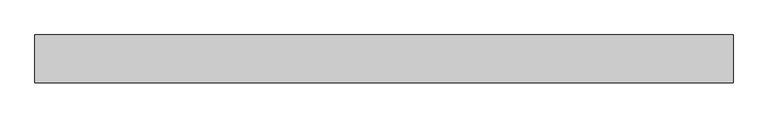
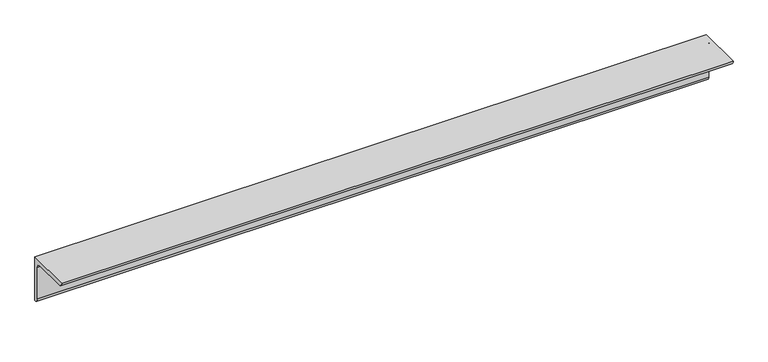
"""IFC4 building model written with IfcOpenShell, lengths in millimetres: member geometry, 0912_Steel Framing_L-KSD3502 : H_SB_AR_S03_L-130x130x12_HBR3."""

import ifcopenshell
import ifcopenshell.guid

model = None  # the IFC model being written
_history = None  # IfcOwnerHistory: only IFC2X3 demands one
_inside = {}  # id of a spatial element -> (the spatial element, [elements in it])
_under = {}  # id of a project, library or spatial element -> (it, [spatial elements below it])
_declared = {}  # id of a project -> (the project, [libraries it declares])
_typed = {}  # id of a type object -> (the type object, [elements of that type])
_made_of = {}  # id of a material, layer set ... -> (it, [elements and type objects made of it])


def new_model(schema):
    """Start an empty IFC model of exactly this schema.

    Asked for "IFC4X3", IfcOpenShell would pick the latest addendum, in which some entities
    have other attributes; the version numbers below select the first issue.
    IFC2X3 requires an IfcOwnerHistory on every rooted entity: one is made here for all.
    """
    global model, _history
    if schema == "IFC4X3":
        model = ifcopenshell.file(schema_version=(4, 3, 0, 0))
    else:
        model = ifcopenshell.file(schema=schema)
    _inside.clear()
    _under.clear()
    _declared.clear()
    _typed.clear()
    _made_of.clear()
    _history = None
    if model.schema == "IFC2X3":
        org = make("IfcOrganization", Name="unknown")
        user = make(
            "IfcPersonAndOrganization",
            ThePerson=make("IfcPerson", FamilyName="unknown"),
            TheOrganization=org,
        )
        app = make(
            "IfcApplication",
            ApplicationDeveloper=org,
            Version="unknown",
            ApplicationFullName="unknown",
            ApplicationIdentifier="unknown",
        )
        _history = make(
            "IfcOwnerHistory",
            OwningUser=user,
            OwningApplication=app,
            ChangeAction="ADDED",
            CreationDate=0,
        )
    return model


def make(cls, **values):
    """One entity of the class cls with the attributes given. An attribute that is None is left unset."""
    return model.create_entity(
        cls, **{name: value for name, value in values.items() if value is not None}
    )


def rooted(cls, **values):
    """An entity with a GlobalId (a new one), such as an element, a storey or a relation."""
    return make(cls, GlobalId=ifcopenshell.guid.new(), OwnerHistory=_history, **values)


def si_unit(unit_type, name, prefix=None):
    """IfcSIUnit, for example si_unit("LENGTHUNIT", "METRE", prefix="MILLI")."""
    return make("IfcSIUnit", UnitType=unit_type, Prefix=prefix, Name=name)


def assignment(units):
    """IfcUnitAssignment: the units of a project."""
    return None if units is None else make("IfcUnitAssignment", Units=units)


def point(xyz):
    """IfcCartesianPoint."""
    return None if xyz is None else make("IfcCartesianPoint", Coordinates=xyz)


def direction(xyz):
    """IfcDirection."""
    return None if xyz is None else make("IfcDirection", DirectionRatios=xyz)


def frame(location, z_axis=None, x_axis=None):
    """IfcAxis2Placement3D, a coordinate frame: its origin and axes. An axis left out is left unset."""
    return make(
        "IfcAxis2Placement3D",
        Location=point(location),
        Axis=direction(z_axis),
        RefDirection=direction(x_axis),
    )


def frame_2d(location, x_axis=None):
    """IfcAxis2Placement2D, a coordinate frame in the plane: its origin and x axis."""
    return make(
        "IfcAxis2Placement2D", Location=point(location), RefDirection=direction(x_axis)
    )


def origin():
    """The frame at (0, 0, 0) with its axes left unset."""
    return frame((0.0, 0.0, 0.0))


def place(relative_to, where):
    """IfcLocalPlacement: puts the frame where relative to a parent placement (None: the world)."""
    return make(
        "IfcLocalPlacement", PlacementRelTo=relative_to, RelativePlacement=where
    )


def context(
    kind, dimensions, precision=None, world=None, true_north=None, identifier=None
):
    """IfcGeometricRepresentationContext, for example the 3D "Model" context."""
    return make(
        "IfcGeometricRepresentationContext",
        ContextIdentifier=identifier,
        ContextType=kind,
        CoordinateSpaceDimension=dimensions,
        Precision=precision,
        WorldCoordinateSystem=world,
        TrueNorth=true_north,
    )


def project(units=None, contexts=None):
    """IfcProject with its units and contexts."""
    return rooted(
        "IfcProject",
        Name="project",
        RepresentationContexts=contexts,
        UnitsInContext=assignment(units),
    )


def spatial(cls, under=None, at=None, **own):
    """A site, building, storey or space (cls), placed at a placement, below another one or the project."""
    s = rooted(cls, ObjectPlacement=at, **own)
    if under is not None:
        _under.setdefault(under.id(), (under, []))[1].append(s)
    return s


def polyline(points):
    """IfcPolyline through the points."""
    return make("IfcPolyline", Points=[point(p) for p in points])


def circle_curve(where, radius):
    """IfcCircle in the frame where."""
    return make("IfcCircle", Position=where, Radius=radius)


def trimmed(basis, trim1, trim2, sense, master):
    """IfcTrimmedCurve: the piece of a basis curve between two trims."""
    return make(
        "IfcTrimmedCurve",
        BasisCurve=basis,
        Trim1=trim1,
        Trim2=trim2,
        SenseAgreement=sense,
        MasterRepresentation=master,
    )


def segment(curve, same_sense, transition):
    """IfcCompositeCurveSegment."""
    return make(
        "IfcCompositeCurveSegment",
        Transition=transition,
        SameSense=same_sense,
        ParentCurve=curve,
    )


def composite_curve(segments, self_intersect=None):
    """IfcCompositeCurve: segments joined end to end."""
    return make("IfcCompositeCurve", Segments=segments, SelfIntersect=self_intersect)


def outline(outer, holes=None, kind="AREA"):
    """IfcArbitraryClosedProfileDef: a profile drawn as a closed curve; with holes, ...WithVoids."""
    if holes is None:
        return make("IfcArbitraryClosedProfileDef", ProfileType=kind, OuterCurve=outer)
    return make(
        "IfcArbitraryProfileDefWithVoids",
        ProfileType=kind,
        OuterCurve=outer,
        InnerCurves=holes,
    )


def extrude(swept, where, along, depth):
    """IfcExtrudedAreaSolid: the profile swept, set in the frame where, extruded along a direction by depth."""
    return make(
        "IfcExtrudedAreaSolid",
        SweptArea=swept,
        Position=where,
        ExtrudedDirection=direction(along),
        Depth=depth,
    )


def shape(context_of_items, identifier, shape_type, items):
    """IfcShapeRepresentation: the items that make up one representation, for example the "Body"."""
    return make(
        "IfcShapeRepresentation",
        ContextOfItems=context_of_items,
        RepresentationIdentifier=identifier,
        RepresentationType=shape_type,
        Items=items,
    )


def source(mapping_origin, context_of_items, identifier, shape_type, items):
    """IfcRepresentationMap: a shape defined once, which mapped items show again and again."""
    return make(
        "IfcRepresentationMap",
        MappingOrigin=mapping_origin,
        MappedRepresentation=shape(context_of_items, identifier, shape_type, items),
    )


def transform(
    local_origin,
    x_axis=None,
    y_axis=None,
    z_axis=None,
    scale=None,
    scale2=None,
    scale3=None,
    uniform=True,
):
    """IfcCartesianTransformationOperator3D, or its non-uniform kind. x_axis, y_axis, z_axis: its Axis1, 2, 3."""
    if uniform:
        return make(
            "IfcCartesianTransformationOperator3D",
            Axis1=direction(x_axis),
            Axis2=direction(y_axis),
            LocalOrigin=point(local_origin),
            Scale=scale,
            Axis3=direction(z_axis),
        )
    return make(
        "IfcCartesianTransformationOperator3DnonUniform",
        Axis1=direction(x_axis),
        Axis2=direction(y_axis),
        LocalOrigin=point(local_origin),
        Scale=scale,
        Axis3=direction(z_axis),
        Scale2=scale2,
        Scale3=scale3,
    )


def mapped(mapping_source, mapping_target):
    """IfcMappedItem: shows the shape of a source again, moved by a transform."""
    return make(
        "IfcMappedItem", MappingSource=mapping_source, MappingTarget=mapping_target
    )


def made_of(thing, what):
    """Note that an element or type object is made of a material, layer set ...; save() writes the relation."""
    if what is not None:
        _made_of.setdefault(what.id(), (what, []))[1].append(thing)
    return thing


def element(
    cls,
    number,
    at=None,
    inside=None,
    cuts=None,
    type_object=None,
    material=None,
    context=None,
    identifier="Body",
    shape_type=None,
    held_by="IfcProductDefinitionShape",
    body=None,
    shapes=None,
    **own,
):
    """One element of the class cls, such as IfcWall. Its Tag is "e" and its number.

    at: its placement. inside: the storey or other place that contains it. cuts: it is an
    opening in that element (IfcRelVoidsElement). A single representation is given by context,
    identifier, shape_type and body (its items); several are given by shapes. held_by: the class
    of the entity that holds the representations. save() writes the other relations.
    """
    e = rooted(cls, Tag="e%d" % number, ObjectPlacement=at, **own)
    if body is not None:
        shapes = [shape(context, identifier, shape_type, body)]
    if shapes is not None:
        e.Representation = make(held_by, Representations=shapes)
    if inside is not None:
        _inside.setdefault(inside.id(), (inside, []))[1].append(e)
    if cuts is not None:
        rooted(
            "IfcRelVoidsElement", RelatingBuildingElement=cuts, RelatedOpeningElement=e
        )
    if type_object is not None:
        _typed.setdefault(type_object.id(), (type_object, []))[1].append(e)
    return made_of(e, material)


def aggregate(whole, parts):
    """IfcRelAggregates: a whole, such as a stair, and the parts it consists of."""
    return rooted("IfcRelAggregates", RelatingObject=whole, RelatedObjects=parts)


def save(model, path):
    """Write the relations noted so far, then the file.

    IfcRelAggregates (storeys below a building ...), IfcRelContainedInSpatialStructure (elements
    in a storey), IfcRelDefinesByType, IfcRelAssociatesMaterial and IfcRelDeclares: one each for
    every whole, place, type object, material and project.
    """
    for whole, parts in _under.values():
        aggregate(whole, parts)
    for where, things in _inside.values():
        rooted(
            "IfcRelContainedInSpatialStructure",
            RelatedElements=things,
            RelatingStructure=where,
        )
    for kind, things in _typed.values():
        rooted("IfcRelDefinesByType", RelatedObjects=things, RelatingType=kind)
    for what, things in _made_of.values():
        rooted("IfcRelAssociatesMaterial", RelatedObjects=things, RelatingMaterial=what)
    for by, libraries in _declared.values():
        rooted("IfcRelDeclares", RelatingContext=by, RelatedDefinitions=libraries)
    model.write(path)


def member_eefd757e(model_context):
    return source(origin(), model_context, "Body", "SweptSolid", [
        extrude(outline(composite_curve([segment(polyline([(36.4, 36.4), (36.4, -93.6)]), True, "CONTINUOUS"), segment(trimmed(circle_curve(frame_2d((36.4, -81.6)), 12.0), [point((36.4, -93.6))], [point((24.4, -81.6))], False, "CARTESIAN"), True, "CONTINUOUS"), segment(polyline([(24.4, -81.6), (24.4, 12.4)]), True, "CONTINUOUS"), segment(trimmed(circle_curve(frame_2d((12.4, 12.4)), 12.0), [point((24.4, 12.4))], [point((12.4, 24.4))], True, "CARTESIAN"), True, "CONTINUOUS"), segment(polyline([(12.4, 24.4), (-81.6, 24.4)]), True, "CONTINUOUS"), segment(trimmed(circle_curve(frame_2d((-81.6, 36.4)), 12.0), [point((-81.6, 24.4))], [point((-93.6, 36.4))], False, "CARTESIAN"), True, "CONTINUOUS"), segment(polyline([(-93.6, 36.4), (36.4, 36.4)]), True, "CONTINUOUS")], self_intersect=False)), frame((-885.3576412, 0.0, 0.0), z_axis=(1.0, 0.0, 0.0), x_axis=(0.0, 1.0, 0.0)), (0.0, 0.0, 1.0), 1889.881949),
    ])


if __name__ == "__main__":
    model = new_model("IFC4")
    model_context = context("Model", 3, world=origin())
    ifc_project = project(units=[si_unit("LENGTHUNIT", "METRE", prefix="MILLI")], contexts=[model_context])
    site = spatial("IfcSite", under=ifc_project)
    building = spatial("IfcBuilding", under=site)
    placement = place(None, origin())
    member_shape = member_eefd757e(model_context)
    element("IfcMember", 1, ObjectType="0912_Steel Framing_L-KSD3502 : H_SB_AR_S03_L-130x130x12_HBR3", at=placement, inside=building, context=model_context, shape_type="MappedRepresentation", body=[
        mapped(member_shape, transform((0.0, 0.0, 0.0), x_axis=(1.0, 0.0, 0.0), y_axis=(0.0, 1.0, 0.0), z_axis=(0.0, 0.0, 1.0))),
    ])
    save(model, "model.ifc")

# Revit data of these elements
# Type "0912_Steel Framing_L-KSD3502 : H_SB_AR_S03_L-130x130x12_HBR3"
#   k = 25 mm
#   Perimeter = 0.52 m²/m
#   Nominal Weight = 23.40 kgf/m
#   Length [instance default] = 1000 mm
#   b = 130 mm
#   d = 130 mm
#   t = 12 mm
#   x = 36.4 mm
#   y = 36.4 mm
#   A = 2976.00 m²
#   Structural Material [instance default] = Steel, 45-345
# Element 1 (IfcMember, "0912_Steel Framing_L-KSD3502 : H_SB_AR_S03_L-130x130x12_HBR3")
#   Structural Material = Steel ASTM A36
#   Materials on its faces: "Steel ASTM A36"
# Materials
#   "Steel, 45-345": class "Metal", colour RGB 189 187 185, transparency 0, Description = "Steel 345 MPa", Cost = 0
#   "Steel ASTM A36": class "Metal", colour RGB 199 199 199, transparency 0, Description = "Structural steel, ASTM A36 Grade B, mill finish", Cost = 0
